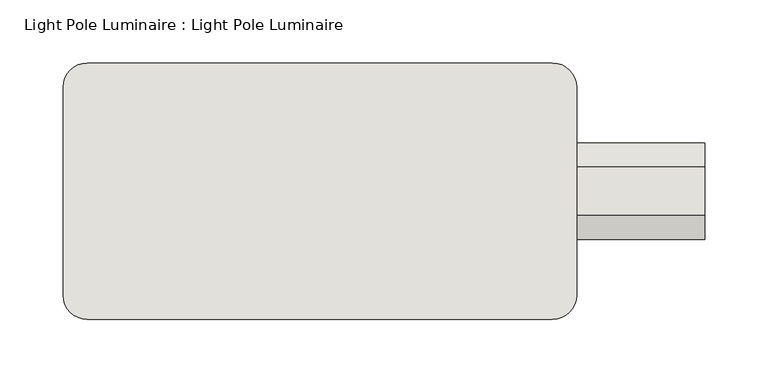
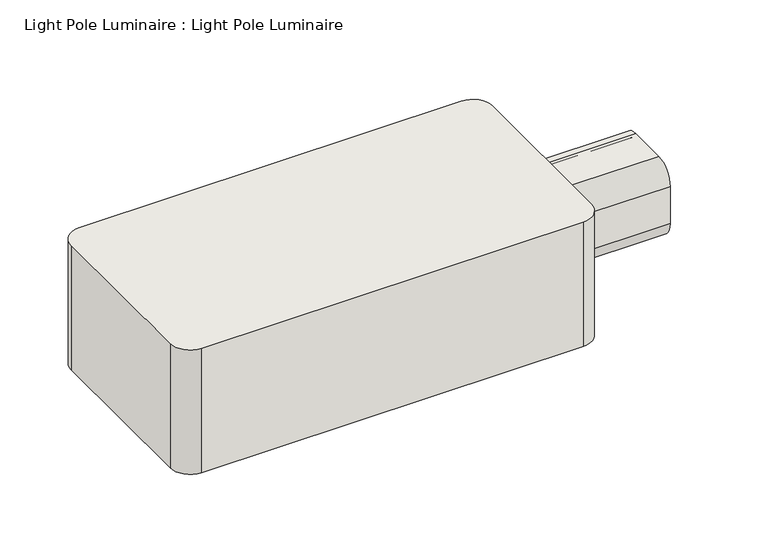
"""IFC4 building model written with IfcOpenShell, lengths in millimetres: wall geometry, Light Pole Luminaire : Light Pole Luminaire."""

import ifcopenshell
import ifcopenshell.guid

model = None  # the IFC model being written
_history = None  # IfcOwnerHistory: only IFC2X3 demands one
_inside = {}  # id of a spatial element -> (the spatial element, [elements in it])
_under = {}  # id of a project, library or spatial element -> (it, [spatial elements below it])
_declared = {}  # id of a project -> (the project, [libraries it declares])
_typed = {}  # id of a type object -> (the type object, [elements of that type])
_made_of = {}  # id of a material, layer set ... -> (it, [elements and type objects made of it])


def new_model(schema):
    """Start an empty IFC model of exactly this schema.

    Asked for "IFC4X3", IfcOpenShell would pick the latest addendum, in which some entities
    have other attributes; the version numbers below select the first issue.
    IFC2X3 requires an IfcOwnerHistory on every rooted entity: one is made here for all.
    """
    global model, _history
    if schema == "IFC4X3":
        model = ifcopenshell.file(schema_version=(4, 3, 0, 0))
    else:
        model = ifcopenshell.file(schema=schema)
    _inside.clear()
    _under.clear()
    _declared.clear()
    _typed.clear()
    _made_of.clear()
    _history = None
    if model.schema == "IFC2X3":
        org = make("IfcOrganization", Name="unknown")
        user = make(
            "IfcPersonAndOrganization",
            ThePerson=make("IfcPerson", FamilyName="unknown"),
            TheOrganization=org,
        )
        app = make(
            "IfcApplication",
            ApplicationDeveloper=org,
            Version="unknown",
            ApplicationFullName="unknown",
            ApplicationIdentifier="unknown",
        )
        _history = make(
            "IfcOwnerHistory",
            OwningUser=user,
            OwningApplication=app,
            ChangeAction="ADDED",
            CreationDate=0,
        )
    return model


def make(cls, **values):
    """One entity of the class cls with the attributes given. An attribute that is None is left unset."""
    return model.create_entity(
        cls, **{name: value for name, value in values.items() if value is not None}
    )


def rooted(cls, **values):
    """An entity with a GlobalId (a new one), such as an element, a storey or a relation."""
    return make(cls, GlobalId=ifcopenshell.guid.new(), OwnerHistory=_history, **values)


def si_unit(unit_type, name, prefix=None):
    """IfcSIUnit, for example si_unit("LENGTHUNIT", "METRE", prefix="MILLI")."""
    return make("IfcSIUnit", UnitType=unit_type, Prefix=prefix, Name=name)


def assignment(units):
    """IfcUnitAssignment: the units of a project."""
    return None if units is None else make("IfcUnitAssignment", Units=units)


def point(xyz):
    """IfcCartesianPoint."""
    return None if xyz is None else make("IfcCartesianPoint", Coordinates=xyz)


def direction(xyz):
    """IfcDirection."""
    return None if xyz is None else make("IfcDirection", DirectionRatios=xyz)


def frame(location, z_axis=None, x_axis=None):
    """IfcAxis2Placement3D, a coordinate frame: its origin and axes. An axis left out is left unset."""
    return make(
        "IfcAxis2Placement3D",
        Location=point(location),
        Axis=direction(z_axis),
        RefDirection=direction(x_axis),
    )


def frame_2d(location, x_axis=None):
    """IfcAxis2Placement2D, a coordinate frame in the plane: its origin and x axis."""
    return make(
        "IfcAxis2Placement2D", Location=point(location), RefDirection=direction(x_axis)
    )


def origin():
    """The frame at (0, 0, 0) with its axes left unset."""
    return frame((0.0, 0.0, 0.0))


def place(relative_to, where):
    """IfcLocalPlacement: puts the frame where relative to a parent placement (None: the world)."""
    return make(
        "IfcLocalPlacement", PlacementRelTo=relative_to, RelativePlacement=where
    )


def context(
    kind, dimensions, precision=None, world=None, true_north=None, identifier=None
):
    """IfcGeometricRepresentationContext, for example the 3D "Model" context."""
    return make(
        "IfcGeometricRepresentationContext",
        ContextIdentifier=identifier,
        ContextType=kind,
        CoordinateSpaceDimension=dimensions,
        Precision=precision,
        WorldCoordinateSystem=world,
        TrueNorth=true_north,
    )


def project(units=None, contexts=None):
    """IfcProject with its units and contexts."""
    return rooted(
        "IfcProject",
        Name="project",
        RepresentationContexts=contexts,
        UnitsInContext=assignment(units),
    )


def spatial(cls, under=None, at=None, **own):
    """A site, building, storey or space (cls), placed at a placement, below another one or the project."""
    s = rooted(cls, ObjectPlacement=at, **own)
    if under is not None:
        _under.setdefault(under.id(), (under, []))[1].append(s)
    return s


def polyline(points):
    """IfcPolyline through the points."""
    return make("IfcPolyline", Points=[point(p) for p in points])


def circle_curve(where, radius):
    """IfcCircle in the frame where."""
    return make("IfcCircle", Position=where, Radius=radius)


def trimmed(basis, trim1, trim2, sense, master):
    """IfcTrimmedCurve: the piece of a basis curve between two trims."""
    return make(
        "IfcTrimmedCurve",
        BasisCurve=basis,
        Trim1=trim1,
        Trim2=trim2,
        SenseAgreement=sense,
        MasterRepresentation=master,
    )


def segment(curve, same_sense, transition):
    """IfcCompositeCurveSegment."""
    return make(
        "IfcCompositeCurveSegment",
        Transition=transition,
        SameSense=same_sense,
        ParentCurve=curve,
    )


def composite_curve(segments, self_intersect=None):
    """IfcCompositeCurve: segments joined end to end."""
    return make("IfcCompositeCurve", Segments=segments, SelfIntersect=self_intersect)


def outline(outer, holes=None, kind="AREA"):
    """IfcArbitraryClosedProfileDef: a profile drawn as a closed curve; with holes, ...WithVoids."""
    if holes is None:
        return make("IfcArbitraryClosedProfileDef", ProfileType=kind, OuterCurve=outer)
    return make(
        "IfcArbitraryProfileDefWithVoids",
        ProfileType=kind,
        OuterCurve=outer,
        InnerCurves=holes,
    )


def extrude(swept, where, along, depth):
    """IfcExtrudedAreaSolid: the profile swept, set in the frame where, extruded along a direction by depth."""
    return make(
        "IfcExtrudedAreaSolid",
        SweptArea=swept,
        Position=where,
        ExtrudedDirection=direction(along),
        Depth=depth,
    )


def shape(context_of_items, identifier, shape_type, items):
    """IfcShapeRepresentation: the items that make up one representation, for example the "Body"."""
    return make(
        "IfcShapeRepresentation",
        ContextOfItems=context_of_items,
        RepresentationIdentifier=identifier,
        RepresentationType=shape_type,
        Items=items,
    )


def source(mapping_origin, context_of_items, identifier, shape_type, items):
    """IfcRepresentationMap: a shape defined once, which mapped items show again and again."""
    return make(
        "IfcRepresentationMap",
        MappingOrigin=mapping_origin,
        MappedRepresentation=shape(context_of_items, identifier, shape_type, items),
    )


def transform(
    local_origin,
    x_axis=None,
    y_axis=None,
    z_axis=None,
    scale=None,
    scale2=None,
    scale3=None,
    uniform=True,
):
    """IfcCartesianTransformationOperator3D, or its non-uniform kind. x_axis, y_axis, z_axis: its Axis1, 2, 3."""
    if uniform:
        return make(
            "IfcCartesianTransformationOperator3D",
            Axis1=direction(x_axis),
            Axis2=direction(y_axis),
            LocalOrigin=point(local_origin),
            Scale=scale,
            Axis3=direction(z_axis),
        )
    return make(
        "IfcCartesianTransformationOperator3DnonUniform",
        Axis1=direction(x_axis),
        Axis2=direction(y_axis),
        LocalOrigin=point(local_origin),
        Scale=scale,
        Axis3=direction(z_axis),
        Scale2=scale2,
        Scale3=scale3,
    )


def mapped(mapping_source, mapping_target):
    """IfcMappedItem: shows the shape of a source again, moved by a transform."""
    return make(
        "IfcMappedItem", MappingSource=mapping_source, MappingTarget=mapping_target
    )


def made_of(thing, what):
    """Note that an element or type object is made of a material, layer set ...; save() writes the relation."""
    if what is not None:
        _made_of.setdefault(what.id(), (what, []))[1].append(thing)
    return thing


def element(
    cls,
    number,
    at=None,
    inside=None,
    cuts=None,
    type_object=None,
    material=None,
    context=None,
    identifier="Body",
    shape_type=None,
    held_by="IfcProductDefinitionShape",
    body=None,
    shapes=None,
    **own,
):
    """One element of the class cls, such as IfcWall. Its Tag is "e" and its number.

    at: its placement. inside: the storey or other place that contains it. cuts: it is an
    opening in that element (IfcRelVoidsElement). A single representation is given by context,
    identifier, shape_type and body (its items); several are given by shapes. held_by: the class
    of the entity that holds the representations. save() writes the other relations.
    """
    e = rooted(cls, Tag="e%d" % number, ObjectPlacement=at, **own)
    if body is not None:
        shapes = [shape(context, identifier, shape_type, body)]
    if shapes is not None:
        e.Representation = make(held_by, Representations=shapes)
    if inside is not None:
        _inside.setdefault(inside.id(), (inside, []))[1].append(e)
    if cuts is not None:
        rooted(
            "IfcRelVoidsElement", RelatingBuildingElement=cuts, RelatedOpeningElement=e
        )
    if type_object is not None:
        _typed.setdefault(type_object.id(), (type_object, []))[1].append(e)
    return made_of(e, material)


def aggregate(whole, parts):
    """IfcRelAggregates: a whole, such as a stair, and the parts it consists of."""
    return rooted("IfcRelAggregates", RelatingObject=whole, RelatedObjects=parts)


def save(model, path):
    """Write the relations noted so far, then the file.

    IfcRelAggregates (storeys below a building ...), IfcRelContainedInSpatialStructure (elements
    in a storey), IfcRelDefinesByType, IfcRelAssociatesMaterial and IfcRelDeclares: one each for
    every whole, place, type object, material and project.
    """
    for whole, parts in _under.values():
        aggregate(whole, parts)
    for where, things in _inside.values():
        rooted(
            "IfcRelContainedInSpatialStructure",
            RelatedElements=things,
            RelatingStructure=where,
        )
    for kind, things in _typed.values():
        rooted("IfcRelDefinesByType", RelatedObjects=things, RelatingType=kind)
    for what, things in _made_of.values():
        rooted("IfcRelAssociatesMaterial", RelatedObjects=things, RelatingMaterial=what)
    for by, libraries in _declared.values():
        rooted("IfcRelDeclares", RelatingContext=by, RelatedDefinitions=libraries)
    model.write(path)


def light_pole_luminaire_light_pole_luminaire_7b1519b5(model_context):
    return source(origin(), model_context, "Body", "SweptSolid", [
        extrude(outline(composite_curve([segment(trimmed(circle_curve(frame_2d((39156.0181437, 683.2325707)), 19.05), [point((39156.0181437, 702.2825707))], [point((39175.0681437, 683.2325707))], False, "CARTESIAN"), True, "CONTINUOUS"), segment(polyline([(39175.0681437, 683.2325707), (39175.0681437, 518.1325707)]), True, "CONTINUOUS"), segment(trimmed(circle_curve(frame_2d((39156.0181437, 518.1325707)), 19.05), [point((39175.0681437, 518.1325707))], [point((39156.0181437, 499.0825707))], False, "CARTESIAN"), True, "CONTINUOUS"), segment(polyline([(39156.0181437, 499.0825707), (38787.7181437, 499.0825707)]), True, "CONTINUOUS"), segment(trimmed(circle_curve(frame_2d((38787.7181437, 518.1325707)), 19.05), [point((38787.7181437, 499.0825707))], [point((38768.6681437, 518.1325707))], False, "CARTESIAN"), True, "CONTINUOUS"), segment(polyline([(38768.6681437, 518.1325707), (38768.6681437, 683.2325707)]), True, "CONTINUOUS"), segment(trimmed(circle_curve(frame_2d((38787.7181437, 683.2325707)), 19.05), [point((38768.6681437, 683.2325707))], [point((38787.7181437, 702.2825707))], False, "CARTESIAN"), True, "CONTINUOUS"), segment(polyline([(38787.7181437, 702.2825707), (39156.0181437, 702.2825707)]), True, "CONTINUOUS")], self_intersect=False)), frame((0.0, 0.0, 8671.0346173), z_axis=(0.0, 0.0, 1.0), x_axis=(1.0, 0.0, 0.0)), (0.0, 0.0, 1.0), 127.0),
        extrude(outline(composite_curve([segment(trimmed(circle_curve(frame_2d((581.6325707, 8753.5846173)), 19.05), [point((562.5825707, 8753.5846173))], [point((581.6325707, 8772.6346173))], False, "CARTESIAN"), True, "CONTINUOUS"), segment(polyline([(581.6325707, 8772.6346173), (619.7325707, 8772.6346173)]), True, "CONTINUOUS"), segment(trimmed(circle_curve(frame_2d((619.7325707, 8753.5846173)), 19.05), [point((619.7325707, 8772.6346173))], [point((638.7825707, 8753.5846173))], False, "CARTESIAN"), True, "CONTINUOUS"), segment(polyline([(638.7825707, 8753.5846173), (638.7825707, 8715.4846173)]), True, "CONTINUOUS"), segment(trimmed(circle_curve(frame_2d((619.7325707, 8715.4846173)), 19.05), [point((638.7825707, 8715.4846173))], [point((619.7325707, 8696.4346173))], False, "CARTESIAN"), True, "CONTINUOUS"), segment(polyline([(619.7325707, 8696.4346173), (581.6325707, 8696.4346173)]), True, "CONTINUOUS"), segment(trimmed(circle_curve(frame_2d((581.6325707, 8715.4846173)), 19.05), [point((581.6325707, 8696.4346173))], [point((562.5825707, 8715.4846173))], False, "CARTESIAN"), True, "CONTINUOUS"), segment(polyline([(562.5825707, 8715.4846173), (562.5825707, 8753.5846173)]), True, "CONTINUOUS")], self_intersect=False), holes=[composite_curve([segment(polyline([(619.7325707, 8766.2846173), (581.6325707, 8766.2846173)]), True, "CONTINUOUS"), segment(trimmed(circle_curve(frame_2d((581.6325707, 8753.5846173)), 12.7), [point((581.6325707, 8766.2846173))], [point((568.9325707, 8753.5846173))], True, "CARTESIAN"), True, "CONTINUOUS"), segment(polyline([(568.9325707, 8753.5846173), (568.9325707, 8715.4846173)]), True, "CONTINUOUS"), segment(trimmed(circle_curve(frame_2d((581.6325707, 8715.4846173)), 12.7), [point((568.9325707, 8715.4846173))], [point((581.6325707, 8702.7846173))], True, "CARTESIAN"), True, "CONTINUOUS"), segment(polyline([(581.6325707, 8702.7846173), (619.7325707, 8702.7846173)]), True, "CONTINUOUS"), segment(trimmed(circle_curve(frame_2d((619.7325707, 8715.4846173)), 12.7), [point((619.7325707, 8702.7846173))], [point((632.4325707, 8715.4846173))], True, "CARTESIAN"), True, "CONTINUOUS"), segment(polyline([(632.4325707, 8715.4846173), (632.4325707, 8753.5846173)]), True, "CONTINUOUS"), segment(trimmed(circle_curve(frame_2d((619.7325707, 8753.5846173)), 12.7), [point((632.4325707, 8753.5846173))], [point((619.7325707, 8766.2846173))], True, "CARTESIAN"), True, "CONTINUOUS")], self_intersect=False)]), frame((39175.0681437, 0.0, 0.0), z_axis=(1.0, 0.0, 0.0), x_axis=(0.0, 1.0, 0.0)), (0.0, 0.0, 1.0), 101.6),
    ])


if __name__ == "__main__":
    model = new_model("IFC4")
    model_context = context("Model", 3, world=origin())
    ifc_project = project(units=[si_unit("LENGTHUNIT", "METRE", prefix="MILLI")], contexts=[model_context])
    site = spatial("IfcSite", under=ifc_project)
    building = spatial("IfcBuilding", under=site)
    placement = place(None, origin())
    light_pole_luminaire_light_pole_luminaire_shape = light_pole_luminaire_light_pole_luminaire_7b1519b5(model_context)
    element("IfcWall", 1, ObjectType="Light Pole Luminaire : Light Pole Luminaire", at=placement, inside=building, context=model_context, shape_type="MappedRepresentation", body=[
        mapped(light_pole_luminaire_light_pole_luminaire_shape, transform((0.0, 0.0, 0.0), x_axis=(1.0, 0.0, 0.0), y_axis=(0.0, 1.0, 0.0), z_axis=(0.0, 0.0, 1.0))),
    ])
    save(model, "model.ifc")

# Revit data of these elements
# Element 1 (IfcWall, "Light Pole Luminaire : Light Pole Luminaire")
#   Materials on its faces: "LUMINAIRE HOUSING AS SPECIFIED"
# Materials
#   "LUMINAIRE HOUSING AS SPECIFIED": class "Metal", colour RGB 247 247 247, transparency 0, Cost = 0
